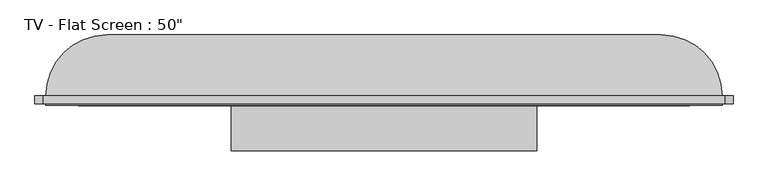
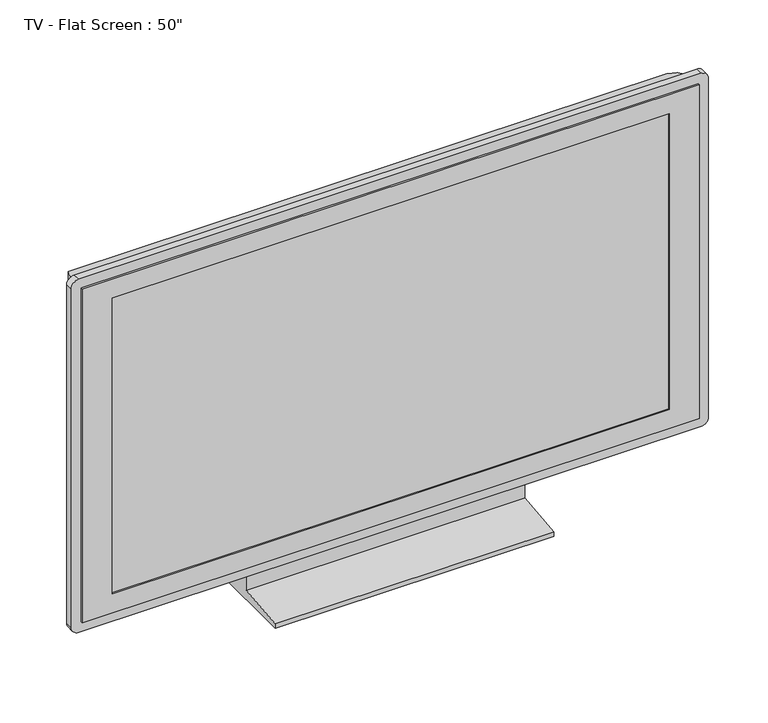
"""IFC4 building model written with IfcOpenShell, lengths in millimetres: furniture geometry."""

import ifcopenshell
import ifcopenshell.guid

model = None  # the IFC model being written
_history = None  # IfcOwnerHistory: only IFC2X3 demands one
_inside = {}  # id of a spatial element -> (the spatial element, [elements in it])
_under = {}  # id of a project, library or spatial element -> (it, [spatial elements below it])
_declared = {}  # id of a project -> (the project, [libraries it declares])
_typed = {}  # id of a type object -> (the type object, [elements of that type])
_made_of = {}  # id of a material, layer set ... -> (it, [elements and type objects made of it])


def new_model(schema):
    """Start an empty IFC model of exactly this schema.

    Asked for "IFC4X3", IfcOpenShell would pick the latest addendum, in which some entities
    have other attributes; the version numbers below select the first issue.
    IFC2X3 requires an IfcOwnerHistory on every rooted entity: one is made here for all.
    """
    global model, _history
    if schema == "IFC4X3":
        model = ifcopenshell.file(schema_version=(4, 3, 0, 0))
    else:
        model = ifcopenshell.file(schema=schema)
    _inside.clear()
    _under.clear()
    _declared.clear()
    _typed.clear()
    _made_of.clear()
    _history = None
    if model.schema == "IFC2X3":
        org = make("IfcOrganization", Name="unknown")
        user = make(
            "IfcPersonAndOrganization",
            ThePerson=make("IfcPerson", FamilyName="unknown"),
            TheOrganization=org,
        )
        app = make(
            "IfcApplication",
            ApplicationDeveloper=org,
            Version="unknown",
            ApplicationFullName="unknown",
            ApplicationIdentifier="unknown",
        )
        _history = make(
            "IfcOwnerHistory",
            OwningUser=user,
            OwningApplication=app,
            ChangeAction="ADDED",
            CreationDate=0,
        )
    return model


def make(cls, **values):
    """One entity of the class cls with the attributes given. An attribute that is None is left unset."""
    return model.create_entity(
        cls, **{name: value for name, value in values.items() if value is not None}
    )


def rooted(cls, **values):
    """An entity with a GlobalId (a new one), such as an element, a storey or a relation."""
    return make(cls, GlobalId=ifcopenshell.guid.new(), OwnerHistory=_history, **values)


def si_unit(unit_type, name, prefix=None):
    """IfcSIUnit, for example si_unit("LENGTHUNIT", "METRE", prefix="MILLI")."""
    return make("IfcSIUnit", UnitType=unit_type, Prefix=prefix, Name=name)


def assignment(units):
    """IfcUnitAssignment: the units of a project."""
    return None if units is None else make("IfcUnitAssignment", Units=units)


def point(xyz):
    """IfcCartesianPoint."""
    return None if xyz is None else make("IfcCartesianPoint", Coordinates=xyz)


def direction(xyz):
    """IfcDirection."""
    return None if xyz is None else make("IfcDirection", DirectionRatios=xyz)


def frame(location, z_axis=None, x_axis=None):
    """IfcAxis2Placement3D, a coordinate frame: its origin and axes. An axis left out is left unset."""
    return make(
        "IfcAxis2Placement3D",
        Location=point(location),
        Axis=direction(z_axis),
        RefDirection=direction(x_axis),
    )


def frame_2d(location, x_axis=None):
    """IfcAxis2Placement2D, a coordinate frame in the plane: its origin and x axis."""
    return make(
        "IfcAxis2Placement2D", Location=point(location), RefDirection=direction(x_axis)
    )


def origin():
    """The frame at (0, 0, 0) with its axes left unset."""
    return frame((0.0, 0.0, 0.0))


def place(relative_to, where):
    """IfcLocalPlacement: puts the frame where relative to a parent placement (None: the world)."""
    return make(
        "IfcLocalPlacement", PlacementRelTo=relative_to, RelativePlacement=where
    )


def context(
    kind, dimensions, precision=None, world=None, true_north=None, identifier=None
):
    """IfcGeometricRepresentationContext, for example the 3D "Model" context."""
    return make(
        "IfcGeometricRepresentationContext",
        ContextIdentifier=identifier,
        ContextType=kind,
        CoordinateSpaceDimension=dimensions,
        Precision=precision,
        WorldCoordinateSystem=world,
        TrueNorth=true_north,
    )


def project(units=None, contexts=None):
    """IfcProject with its units and contexts."""
    return rooted(
        "IfcProject",
        Name="project",
        RepresentationContexts=contexts,
        UnitsInContext=assignment(units),
    )


def spatial(cls, under=None, at=None, **own):
    """A site, building, storey or space (cls), placed at a placement, below another one or the project."""
    s = rooted(cls, ObjectPlacement=at, **own)
    if under is not None:
        _under.setdefault(under.id(), (under, []))[1].append(s)
    return s


def polyline(points):
    """IfcPolyline through the points."""
    return make("IfcPolyline", Points=[point(p) for p in points])


def circle_curve(where, radius):
    """IfcCircle in the frame where."""
    return make("IfcCircle", Position=where, Radius=radius)


def ellipse_curve(where, semi_axis1, semi_axis2):
    """IfcEllipse in the frame where."""
    return make(
        "IfcEllipse", Position=where, SemiAxis1=semi_axis1, SemiAxis2=semi_axis2
    )


def trimmed(basis, trim1, trim2, sense, master):
    """IfcTrimmedCurve: the piece of a basis curve between two trims."""
    return make(
        "IfcTrimmedCurve",
        BasisCurve=basis,
        Trim1=trim1,
        Trim2=trim2,
        SenseAgreement=sense,
        MasterRepresentation=master,
    )


def segment(curve, same_sense, transition):
    """IfcCompositeCurveSegment."""
    return make(
        "IfcCompositeCurveSegment",
        Transition=transition,
        SameSense=same_sense,
        ParentCurve=curve,
    )


def composite_curve(segments, self_intersect=None):
    """IfcCompositeCurve: segments joined end to end."""
    return make("IfcCompositeCurve", Segments=segments, SelfIntersect=self_intersect)


def outline(outer, holes=None, kind="AREA"):
    """IfcArbitraryClosedProfileDef: a profile drawn as a closed curve; with holes, ...WithVoids."""
    if holes is None:
        return make("IfcArbitraryClosedProfileDef", ProfileType=kind, OuterCurve=outer)
    return make(
        "IfcArbitraryProfileDefWithVoids",
        ProfileType=kind,
        OuterCurve=outer,
        InnerCurves=holes,
    )


def extrude(swept, where, along, depth):
    """IfcExtrudedAreaSolid: the profile swept, set in the frame where, extruded along a direction by depth."""
    return make(
        "IfcExtrudedAreaSolid",
        SweptArea=swept,
        Position=where,
        ExtrudedDirection=direction(along),
        Depth=depth,
    )


def faces_of(points, faces, orient=None, outer=None):
    """IfcFace entities. A face is a list of loops; a loop is a list of indices into points, from 0.

    orient and outer hold one flag for each loop. By default every Orientation is true, the
    first loop of a face is its IfcFaceOuterBound and the others are IfcFaceBound.
    """
    made = []
    for i, loops in enumerate(faces):
        bounds = []
        for j, loop in enumerate(loops):
            is_outer = j == 0 if outer is None else outer[i][j]
            bounds.append(
                make(
                    "IfcFaceOuterBound" if is_outer else "IfcFaceBound",
                    Bound=make("IfcPolyLoop", Polygon=[points[k] for k in loop]),
                    Orientation=True if orient is None else orient[i][j],
                )
            )
        made.append(make("IfcFace", Bounds=bounds))
    return made


def faceted_brep(points, faces, orient=None, outer=None, voids=None):
    """IfcFacetedBrep: a solid bounded by flat faces; with voids (closed shells), ...WithVoids."""
    shared = [point(p) for p in points]
    hull = make("IfcClosedShell", CfsFaces=faces_of(shared, faces, orient, outer))
    if voids is None:
        return make("IfcFacetedBrep", Outer=hull)
    return make(
        "IfcFacetedBrepWithVoids",
        Outer=hull,
        Voids=[
            make(cls, CfsFaces=faces_of(shared, fs, o, b)) for cls, fs, o, b in voids
        ],
    )


def shape(context_of_items, identifier, shape_type, items):
    """IfcShapeRepresentation: the items that make up one representation, for example the "Body"."""
    return make(
        "IfcShapeRepresentation",
        ContextOfItems=context_of_items,
        RepresentationIdentifier=identifier,
        RepresentationType=shape_type,
        Items=items,
    )


def source(mapping_origin, context_of_items, identifier, shape_type, items):
    """IfcRepresentationMap: a shape defined once, which mapped items show again and again."""
    return make(
        "IfcRepresentationMap",
        MappingOrigin=mapping_origin,
        MappedRepresentation=shape(context_of_items, identifier, shape_type, items),
    )


def transform(
    local_origin,
    x_axis=None,
    y_axis=None,
    z_axis=None,
    scale=None,
    scale2=None,
    scale3=None,
    uniform=True,
):
    """IfcCartesianTransformationOperator3D, or its non-uniform kind. x_axis, y_axis, z_axis: its Axis1, 2, 3."""
    if uniform:
        return make(
            "IfcCartesianTransformationOperator3D",
            Axis1=direction(x_axis),
            Axis2=direction(y_axis),
            LocalOrigin=point(local_origin),
            Scale=scale,
            Axis3=direction(z_axis),
        )
    return make(
        "IfcCartesianTransformationOperator3DnonUniform",
        Axis1=direction(x_axis),
        Axis2=direction(y_axis),
        LocalOrigin=point(local_origin),
        Scale=scale,
        Axis3=direction(z_axis),
        Scale2=scale2,
        Scale3=scale3,
    )


def mapped(mapping_source, mapping_target):
    """IfcMappedItem: shows the shape of a source again, moved by a transform."""
    return make(
        "IfcMappedItem", MappingSource=mapping_source, MappingTarget=mapping_target
    )


def made_of(thing, what):
    """Note that an element or type object is made of a material, layer set ...; save() writes the relation."""
    if what is not None:
        _made_of.setdefault(what.id(), (what, []))[1].append(thing)
    return thing


def element(
    cls,
    number,
    at=None,
    inside=None,
    cuts=None,
    type_object=None,
    material=None,
    context=None,
    identifier="Body",
    shape_type=None,
    held_by="IfcProductDefinitionShape",
    body=None,
    shapes=None,
    **own,
):
    """One element of the class cls, such as IfcWall. Its Tag is "e" and its number.

    at: its placement. inside: the storey or other place that contains it. cuts: it is an
    opening in that element (IfcRelVoidsElement). A single representation is given by context,
    identifier, shape_type and body (its items); several are given by shapes. held_by: the class
    of the entity that holds the representations. save() writes the other relations.
    """
    e = rooted(cls, Tag="e%d" % number, ObjectPlacement=at, **own)
    if body is not None:
        shapes = [shape(context, identifier, shape_type, body)]
    if shapes is not None:
        e.Representation = make(held_by, Representations=shapes)
    if inside is not None:
        _inside.setdefault(inside.id(), (inside, []))[1].append(e)
    if cuts is not None:
        rooted(
            "IfcRelVoidsElement", RelatingBuildingElement=cuts, RelatedOpeningElement=e
        )
    if type_object is not None:
        _typed.setdefault(type_object.id(), (type_object, []))[1].append(e)
    return made_of(e, material)


def aggregate(whole, parts):
    """IfcRelAggregates: a whole, such as a stair, and the parts it consists of."""
    return rooted("IfcRelAggregates", RelatingObject=whole, RelatedObjects=parts)


def save(model, path):
    """Write the relations noted so far, then the file.

    IfcRelAggregates (storeys below a building ...), IfcRelContainedInSpatialStructure (elements
    in a storey), IfcRelDefinesByType, IfcRelAssociatesMaterial and IfcRelDeclares: one each for
    every whole, place, type object, material and project.
    """
    for whole, parts in _under.values():
        aggregate(whole, parts)
    for where, things in _inside.values():
        rooted(
            "IfcRelContainedInSpatialStructure",
            RelatedElements=things,
            RelatingStructure=where,
        )
    for kind, things in _typed.values():
        rooted("IfcRelDefinesByType", RelatedObjects=things, RelatingType=kind)
    for what, things in _made_of.values():
        rooted("IfcRelAssociatesMaterial", RelatedObjects=things, RelatingMaterial=what)
    for by, libraries in _declared.values():
        rooted("IfcRelDeclares", RelatingContext=by, RelatedDefinitions=libraries)
    model.write(path)


def plane_surface(at):
    """IfcPlane: the flat surface through the origin of the frame at, square to its z axis."""
    return make("IfcPlane", Position=at)


def cylinder_surface(at, radius):
    """IfcCylindricalSurface: all points at the distance radius from the z axis of the frame at."""
    return make("IfcCylindricalSurface", Position=at, Radius=radius)


def advanced_brep(points, edges, surfaces, faces):
    """IfcAdvancedBrep: a solid bounded by faces that lie on surfaces and meet in shared edges.

    An edge is (start, end): straight between two places in points (the first is 0);
    or (start, end, curve); or (start, end, curve, False) where it runs against its curve.
    A face is (place in surfaces, loops), or (place, loops, False) where it looks against
    its surface's normal. A loop lists edges by number (the first is 1), with a minus sign
    where the edge is run from its end to its start. The first loop is the outer one.
    """
    corners = [point(p) for p in points]
    vertices = [make("IfcVertexPoint", VertexGeometry=c) for c in corners]
    made = []
    for start, end, *more in edges:
        made.append(
            make(
                "IfcEdgeCurve",
                EdgeStart=vertices[start],
                EdgeEnd=vertices[end],
                EdgeGeometry=more[0] if more else make("IfcPolyline", Points=[corners[start], corners[end]]),
                SameSense=more[1] if len(more) > 1 else True,
            )
        )
    hull = []
    for where, loops, *sense in faces:
        bounds = []
        for j, loop in enumerate(loops):
            ring = [make("IfcOrientedEdge", EdgeElement=made[abs(k) - 1], Orientation=k > 0) for k in loop]
            bounds.append(
                make(
                    "IfcFaceOuterBound" if j == 0 else "IfcFaceBound",
                    Bound=make("IfcEdgeLoop", EdgeList=ring),
                    Orientation=True,
                )
            )
        hull.append(make("IfcAdvancedFace", Bounds=bounds, FaceSurface=surfaces[where], SameSense=sense[0] if sense else True))
    return make("IfcAdvancedBrep", Outer=make("IfcClosedShell", CfsFaces=hull))


def furniture_fdf74506(model_context):
    return source(origin(), model_context, "Body", "SolidModel", [
        extrude(outline(polyline([(-51.4613764, 80.0), (-1.4613764, 80.0), (48.5386236, 0.0), (-151.4613764, 0.0), (-151.4613764, 10.0), (-51.4613764, 20.0), (-51.4613764, 80.0)])), frame((-280.6636439, 0.0, 0.0), z_axis=(1.0, 0.0, 0.0), x_axis=(0.0, 1.0, 0.0)), (0.0, 0.0, 1.0), 553.4382596),
        faceted_brep([(609.4937454, -69.4613764, 782.6751733), (-617.3827737, -69.4613764, 782.6751733), (-617.3827737, -69.4613764, 80.0), (609.4937454, -69.4613764, 80.0), (-557.3827737, -69.4613764, 742.6751733), (549.4937454, -69.4613764, 742.6751733), (549.4937454, -69.4613764, 120.0), (-557.3827737, -69.4613764, 120.0), (609.4937454, -51.4613764, 782.6751733), (609.4937454, -51.4613764, 80.0), (-617.3827737, -51.4613764, 80.0), (-617.3827737, -51.4613764, 782.6751733), (-557.3827737, -66.4613764, 742.6751733), (-557.3827737, -66.4613764, 120.0), (549.4937454, -66.4613764, 120.0), (549.4937454, -66.4613764, 742.6751733)], [[[0, 1, 2, 3], [4, 5, 6, 7]], [[8, 9, 10, 11]], [[1, 0, 8, 11]], [[2, 1, 11, 10]], [[3, 2, 10, 9]], [[0, 3, 9, 8]], [[12, 13, 14, 15]], [[12, 15, 5, 4]], [[15, 14, 6, 5]], [[14, 13, 7, 6]], [[13, 12, 4, 7]]]),
        extrude(outline(composite_curve([segment(polyline([(802.6751733, 614.4937454), (802.6751733, -622.3827737)]), True, "CONTINUOUS"), segment(trimmed(circle_curve(frame_2d((787.6751733, -622.3827737)), 15.0), [point((802.6751733, -622.3827737))], [point((787.6751733, -637.3827737))], False, "CARTESIAN"), True, "CONTINUOUS"), segment(polyline([(787.6751733, -637.3827737), (75.0, -637.3827737)]), True, "CONTINUOUS"), segment(trimmed(circle_curve(frame_2d((75.0, -622.3827737)), 15.0), [point((75.0, -637.3827737))], [point((60.0, -622.3827737))], False, "CARTESIAN"), True, "CONTINUOUS"), segment(polyline([(60.0, -622.3827737), (60.0, 614.4937454)]), True, "CONTINUOUS"), segment(trimmed(circle_curve(frame_2d((75.0, 614.4937454)), 15.0), [point((60.0, 614.4937454))], [point((75.0, 629.4937454))], False, "CARTESIAN"), True, "CONTINUOUS"), segment(polyline([(75.0, 629.4937454), (787.6751733, 629.4937454)]), True, "CONTINUOUS"), segment(trimmed(circle_curve(frame_2d((787.6751733, 614.4937454)), 15.0), [point((787.6751733, 629.4937454))], [point((802.6751733, 614.4937454))], False, "CARTESIAN"), True, "CONTINUOUS")], self_intersect=False), holes=[polyline([(782.6751733, 609.4937454), (80.0, 609.4937454), (80.0, -617.3827737), (782.6751733, -617.3827737), (782.6751733, 609.4937454)])]), frame((0.0, -66.4613764, 0.0), z_axis=(0.0, 1.0, 0.0), x_axis=(0.0, 0.0, 1.0)), (0.0, 0.0, 1.0), 15.0),
        advanced_brep(
        [(-617.3827737, -51.4613764, 80.0), (609.4937454, -51.4613764, 80.0), (609.4937454, -51.4613764, 782.6751733), (-617.3827737, -51.4613764, 782.6751733), (499.4937454, 58.5386236, 80.0), (-507.3827737, 58.5386236, 80.0), (-507.3827737, 58.5386236, 672.6751733), (499.4937454, 58.5386236, 672.6751733)],
        [
            (0, 1),
            (1, 2),
            (2, 3),
            (3, 0),
            (4, 5),
            (5, 6),
            (6, 7),
            (7, 4),
            (0, 5, circle_curve(frame((-507.3827737, -51.4613764, 80.0), z_axis=(0.0, 0.0, -1.0), x_axis=(-1.0, 0.0, 0.0)), 110.0)),
            (4, 1, circle_curve(frame((499.4937454, -51.4613764, 80.0), z_axis=(0.0, 0.0, -1.0), x_axis=(1.0, 0.0, 0.0)), 110.0)),
            (7, 2, ellipse_curve(frame((499.4937454, -51.4613764, 672.6751733), z_axis=(0.7071067811865475, 0.0, -0.7071067811865475), x_axis=(0.7071067811865474, 0.0, 0.7071067811865476)), 155.5634919, 110.0)),
            (6, 3, ellipse_curve(frame((-507.3827737, -51.4613764, 672.6751733), z_axis=(0.7071067811865475, 0.0, 0.7071067811865475), x_axis=(-0.7071067811865476, 0.0, 0.7071067811865474)), 155.5634919, 110.0)),
        ],
        [
            plane_surface(frame((-617.3827737, -51.4613764, 782.6751733), z_axis=(0.0, -1.0, 0.0), x_axis=(-1.0, 0.0, 0.0))),
            plane_surface(frame((-617.3827737, 58.5386236, 782.6751733), z_axis=(0.0, 1.0, 0.0), x_axis=(1.0, 0.0, 0.0))),
            plane_surface(frame((-617.3827737, -51.4613764, 80.0), z_axis=(0.0, 0.0, -1.0), x_axis=(0.0, 1.0, 0.0))),
            cylinder_surface(frame((499.4937454, -51.4613764, 80.0), z_axis=(0.0, 0.0, 1.0), x_axis=(1.0, 0.0, 0.0)), 110.0),
            cylinder_surface(frame((609.4937454, -51.4613764, 672.6751733), z_axis=(-1.0, 0.0, 0.0), x_axis=(0.0, 0.0, 1.0)), 110.0),
            cylinder_surface(frame((-507.3827737, -51.4613764, 782.6751733), z_axis=(0.0, 0.0, -1.0), x_axis=(-1.0, 0.0, 0.0)), 110.0),
        ],
        [
            (0, [[1, 2, 3, 4]]),
            (1, [[5, 6, 7, 8]]),
            (2, [[-1, 9, -5, 10]]),
            (3, [[11, -2, -10, -8]]),
            (4, [[-11, -7, 12, -3]]),
            (5, [[-12, -6, -9, -4]]),
        ],
    ),
    ])


if __name__ == "__main__":
    model = new_model("IFC4")
    model_context = context("Model", 3, world=origin())
    ifc_project = project(units=[si_unit("LENGTHUNIT", "METRE", prefix="MILLI")], contexts=[model_context])
    site = spatial("IfcSite", under=ifc_project)
    building = spatial("IfcBuilding", under=site)
    placement = place(None, origin())
    furniture_shape = furniture_fdf74506(model_context)
    element("IfcFurniture", 1, ObjectType="TV - Flat Screen : 50\"", at=placement, inside=building, context=model_context, shape_type="MappedRepresentation", body=[
        mapped(furniture_shape, transform((0.0, 0.0, 0.0), x_axis=(1.0, 0.0, 0.0), y_axis=(0.0, 1.0, 0.0), z_axis=(0.0, 0.0, 1.0))),
    ])
    save(model, "model.ifc")

# Revit data of these elements
# Project information
#   Project Issue Date = "Issue Date"
#   Project Status = "Project Status"
#   Client Name = "Owner"
#   Project Address = "Enter address here"
#   Project Name = "Project Name"
#   Project Number = "Project Number"
# Type "TV - Flat Screen : 50\""
#   SinAng = 0' - 0.0193"
#   L = 3' - 7.57782"
#   H = 2' - 0.51477"
#   Thickness = 0' - 4.33071"
#   Diagonal = 4' - 2"
#   CosAng = 0' - 0.03431"
#   Stand [instance default] = yes
# Element 1 (IfcFurniture, "TV - Flat Screen : 50\"")
#   Materials on its faces: "TV - Black", "TV - Glass", "TV - Screen"
# Materials
#   "TV - Black": class "Miscellaneous", colour RGB 49 49 49, transparency 0
#   "TV - Glass": class "Miscellaneous", colour RGB 157 157 157, transparency 0.9
#   "TV - Screen": class "Miscellaneous", colour RGB 0 0 0, transparency 0
